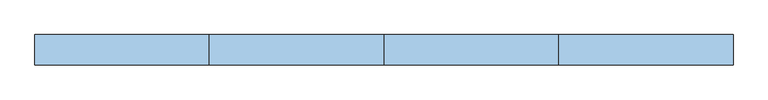
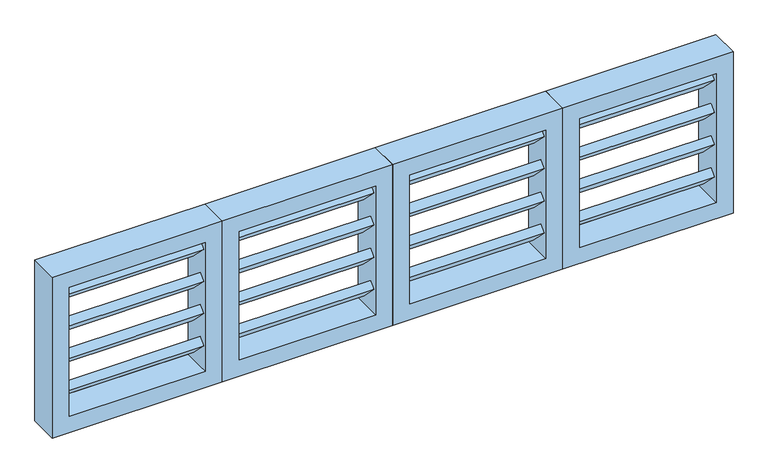
"""IFC4 building model written with IfcOpenShell, lengths in millimetres: window geometry, Elemento Vazado - Veneziana : 4 Módulos."""

from ifc_helpers import new_model, si_unit, frame, origin, place, context, project, spatial, polyline, outline, extrude, source, transform, mapped, element, save


def window_1cea5f9a(model_context):
    return source(origin(), model_context, "Body", "SweptSolid", [
        extrude(outline(polyline([(0.0, -60.0), (0.0, 0.0), (320.0, 0.0), (320.0, -60.0), (0.0, -60.0)])), frame((760.0, -63.5827536, 2699.5955527), z_axis=(0.0, 0.707106781186549, 0.7071067811865461), x_axis=(-1.0, 0.0, 0.0)), (0.0, 0.0, 1.0), 20.0),
        extrude(outline(polyline([(0.0, -60.0), (0.0, 0.0), (320.0, 0.0), (320.0, -60.0), (0.0, -60.0)])), frame((760.0, -63.5827536, 2779.5955527), z_axis=(0.0, 0.7071067811865492, 0.7071067811865458), x_axis=(-1.0, 0.0, 0.0)), (0.0, 0.0, 1.0), 20.0),
        extrude(outline(polyline([(0.0, -60.0), (0.0, 0.0), (320.0, 0.0), (320.0, -60.0), (0.0, -60.0)])), frame((760.0, -63.5827536, 2859.5955527), z_axis=(0.0, 0.7071067811865492, 0.7071067811865459), x_axis=(-1.0, 0.0, 0.0)), (0.0, 0.0, 1.0), 20.0),
        extrude(outline(polyline([(0.0, -60.0), (0.0, 0.0), (320.0, 0.0), (320.0, -60.0), (0.0, -60.0)])), frame((760.0, -63.5827536, 2939.5955527), z_axis=(0.0, 0.707106781186549, 0.7071067811865461), x_axis=(-1.0, 0.0, 0.0)), (0.0, 0.0, 1.0), 20.0),
        extrude(outline(polyline([(3000.0, 800.0), (3000.0, 400.0), (2600.0, 400.0), (2600.0, 800.0), (3000.0, 800.0)]), holes=[polyline([(2960.0, 760.0), (2640.0, 760.0), (2640.0, 440.0), (2960.0, 440.0), (2960.0, 760.0)])]), frame((0.0, -70.0, 0.0), z_axis=(0.0, 1.0, 0.0), x_axis=(0.0, 0.0, 1.0)), (0.0, 0.0, 1.0), 70.0),
        extrude(outline(polyline([(0.0, -60.0), (0.0, 0.0), (320.0, 0.0), (320.0, -60.0), (0.0, -60.0)])), frame((360.0, -63.5827536, 2699.5955527), z_axis=(0.0, 0.707106781186549, 0.7071067811865461), x_axis=(-1.0, 0.0, 0.0)), (0.0, 0.0, 1.0), 20.0),
        extrude(outline(polyline([(0.0, -60.0), (0.0, 0.0), (320.0, 0.0), (320.0, -60.0), (0.0, -60.0)])), frame((360.0, -63.5827536, 2779.5955527), z_axis=(0.0, 0.7071067811865492, 0.7071067811865458), x_axis=(-1.0, 0.0, 0.0)), (0.0, 0.0, 1.0), 20.0),
        extrude(outline(polyline([(0.0, -60.0), (0.0, 0.0), (320.0, 0.0), (320.0, -60.0), (0.0, -60.0)])), frame((360.0, -63.5827536, 2859.5955527), z_axis=(0.0, 0.7071067811865492, 0.7071067811865459), x_axis=(-1.0, 0.0, 0.0)), (0.0, 0.0, 1.0), 20.0),
        extrude(outline(polyline([(0.0, -60.0), (0.0, 0.0), (320.0, 0.0), (320.0, -60.0), (0.0, -60.0)])), frame((360.0, -63.5827536, 2939.5955527), z_axis=(0.0, 0.707106781186549, 0.7071067811865461), x_axis=(-1.0, 0.0, 0.0)), (0.0, 0.0, 1.0), 20.0),
        extrude(outline(polyline([(3000.0, 400.0), (3000.0, 0.0), (2600.0, 0.0), (2600.0, 400.0), (3000.0, 400.0)]), holes=[polyline([(2960.0, 360.0), (2640.0, 360.0), (2640.0, 40.0), (2960.0, 40.0), (2960.0, 360.0)])]), frame((0.0, -70.0, 0.0), z_axis=(0.0, 1.0, 0.0), x_axis=(0.0, 0.0, 1.0)), (0.0, 0.0, 1.0), 70.0),
        extrude(outline(polyline([(0.0, -60.0), (0.0, 0.0), (320.0, 0.0), (320.0, -60.0), (0.0, -60.0)])), frame((-40.0, -63.5827536, 2699.5955527), z_axis=(0.0, 0.707106781186549, 0.7071067811865461), x_axis=(-1.0, 0.0, 0.0)), (0.0, 0.0, 1.0), 20.0),
        extrude(outline(polyline([(0.0, -60.0), (0.0, 0.0), (320.0, 0.0), (320.0, -60.0), (0.0, -60.0)])), frame((-40.0, -63.5827536, 2779.5955527), z_axis=(0.0, 0.7071067811865492, 0.7071067811865458), x_axis=(-1.0, 0.0, 0.0)), (0.0, 0.0, 1.0), 20.0),
        extrude(outline(polyline([(0.0, -60.0), (0.0, 0.0), (320.0, 0.0), (320.0, -60.0), (0.0, -60.0)])), frame((-40.0, -63.5827536, 2859.5955527), z_axis=(0.0, 0.7071067811865492, 0.7071067811865459), x_axis=(-1.0, 0.0, 0.0)), (0.0, 0.0, 1.0), 20.0),
        extrude(outline(polyline([(0.0, -60.0), (0.0, 0.0), (320.0, 0.0), (320.0, -60.0), (0.0, -60.0)])), frame((-40.0, -63.5827536, 2939.5955527), z_axis=(0.0, 0.707106781186549, 0.7071067811865461), x_axis=(-1.0, 0.0, 0.0)), (0.0, 0.0, 1.0), 20.0),
        extrude(outline(polyline([(3000.0, 0.0), (3000.0, -400.0), (2600.0, -400.0), (2600.0, 0.0), (3000.0, 0.0)]), holes=[polyline([(2960.0, -40.0), (2640.0, -40.0), (2640.0, -360.0), (2960.0, -360.0), (2960.0, -40.0)])]), frame((0.0, -70.0, 0.0), z_axis=(0.0, 1.0, 0.0), x_axis=(0.0, 0.0, 1.0)), (0.0, 0.0, 1.0), 70.0),
        extrude(outline(polyline([(0.0, -60.0), (0.0, 0.0), (320.0, 0.0), (320.0, -60.0), (0.0, -60.0)])), frame((-440.0, -63.5827536, 2699.5955527), z_axis=(0.0, 0.707106781186549, 0.7071067811865461), x_axis=(-1.0, 0.0, 0.0)), (0.0, 0.0, 1.0), 20.0),
        extrude(outline(polyline([(0.0, -60.0), (0.0, 0.0), (320.0, 0.0), (320.0, -60.0), (0.0, -60.0)])), frame((-440.0, -63.5827536, 2779.5955527), z_axis=(0.0, 0.7071067811865492, 0.7071067811865458), x_axis=(-1.0, 0.0, 0.0)), (0.0, 0.0, 1.0), 20.0),
        extrude(outline(polyline([(0.0, -60.0), (0.0, 0.0), (320.0, 0.0), (320.0, -60.0), (0.0, -60.0)])), frame((-440.0, -63.5827536, 2859.5955527), z_axis=(0.0, 0.7071067811865492, 0.7071067811865459), x_axis=(-1.0, 0.0, 0.0)), (0.0, 0.0, 1.0), 20.0),
        extrude(outline(polyline([(0.0, -60.0), (0.0, 0.0), (320.0, 0.0), (320.0, -60.0), (0.0, -60.0)])), frame((-440.0, -63.5827536, 2939.5955527), z_axis=(0.0, 0.707106781186549, 0.7071067811865461), x_axis=(-1.0, 0.0, 0.0)), (0.0, 0.0, 1.0), 20.0),
        extrude(outline(polyline([(3000.0, -400.0), (3000.0, -800.0), (2600.0, -800.0), (2600.0, -400.0), (3000.0, -400.0)]), holes=[polyline([(2960.0, -440.0), (2640.0, -440.0), (2640.0, -760.0), (2960.0, -760.0), (2960.0, -440.0)])]), frame((0.0, -70.0, 0.0), z_axis=(0.0, 1.0, 0.0), x_axis=(0.0, 0.0, 1.0)), (0.0, 0.0, 1.0), 70.0),
    ])


if __name__ == "__main__":
    model = new_model("IFC4")
    model_context = context("Model", 3, world=origin())
    ifc_project = project(units=[si_unit("LENGTHUNIT", "METRE", prefix="MILLI")], contexts=[model_context])
    site = spatial("IfcSite", under=ifc_project)
    building = spatial("IfcBuilding", under=site)
    placement = place(None, origin())
    window_shape = window_1cea5f9a(model_context)
    element("IfcWindow", 1, ObjectType="Elemento Vazado - Veneziana : 4 Módulos", at=placement, inside=building, context=model_context, shape_type="MappedRepresentation", body=[
        mapped(window_shape, transform((0.0, 0.0, 0.0), x_axis=(1.0, 0.0, 0.0), y_axis=(0.0, 1.0, 0.0), z_axis=(0.0, 0.0, 1.0))),
    ])
    save(model, "model.ifc")

# Revit data of these elements
# Type "Elemento Vazado - Veneziana : 4 Módulos"
#   Type Mark = ""
#   SINAPI = ""
#   Ref. modular de largura = 40.00 cm
#   Ref. modular de altura = 40.00 cm
#   Módulo Básico M = 10.00 cm
#   Largura de Coordenação Modular CM = 160.00 cm
#   Altura de Coordenação Modular CM = 40.00 cm
#   Height = 40.00 cm
#   Altura Peitoril = 260.00 cm
#   Width = 160.00 cm
#   n° módulos = 4
#   Número de Módulos Básicos nM Largura = 4
#   Número de Módulos Básicos nM Altura = 4
#   Assembly Code = ""
#   Wall Closure = (empty or 0)
